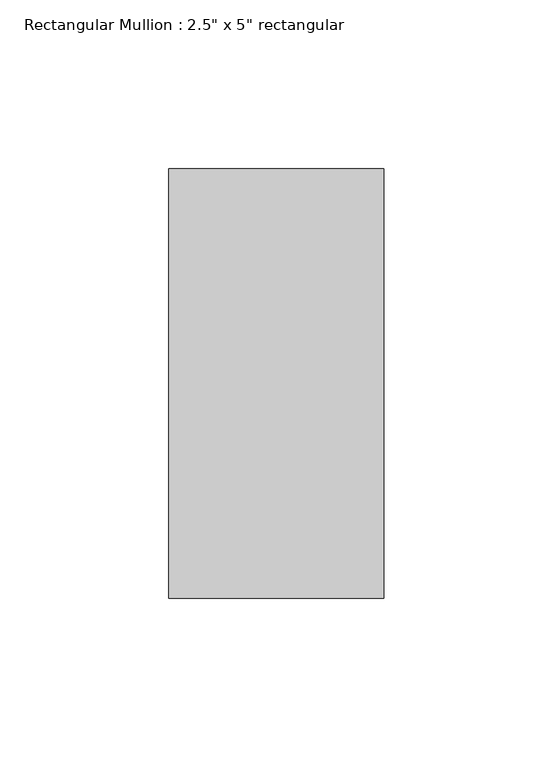
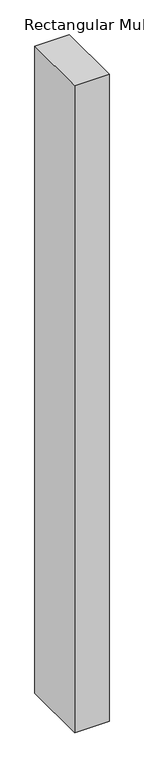
"""IFC4 building model written with IfcOpenShell, lengths in millimetres: member geometry."""

from ifc_helpers import new_model, si_unit, frame, origin, place, context, project, spatial, polyline, outline, extrude, source, transform, mapped, element, save


def member_76223ac8(model_context):
    return source(origin(), model_context, "Body", "SweptSolid", [
        extrude(outline(polyline([(31.75, 63.5), (31.75, -63.5), (-31.75, -63.5), (-31.75, 63.5), (31.75, 63.5)])), frame((0.0, 0.0, -1263.65), z_axis=(0.0, 0.0, 1.0), x_axis=(1.0, 0.0, 0.0)), (0.0, 0.0, 1.0), 1263.65),
    ])


if __name__ == "__main__":
    model = new_model("IFC4")
    model_context = context("Model", 3, world=origin())
    ifc_project = project(units=[si_unit("LENGTHUNIT", "METRE", prefix="MILLI")], contexts=[model_context])
    site = spatial("IfcSite", under=ifc_project)
    building = spatial("IfcBuilding", under=site)
    placement = place(None, origin())
    member_shape = member_76223ac8(model_context)
    element("IfcMember", 1, ObjectType="Rectangular Mullion : 2.5\" x 5\" rectangular", at=placement, inside=building, context=model_context, shape_type="MappedRepresentation", body=[
        mapped(member_shape, transform((0.0, 0.0, 0.0), x_axis=(1.0, 0.0, 0.0), y_axis=(0.0, 1.0, 0.0), z_axis=(0.0, 0.0, 1.0))),
    ])
    save(model, "model.ifc")

# Revit data of these elements
# Type "Rectangular Mullion : 2.5\" x 5\" rectangular"
#   built-in parameter 1007304 = 0.416667 (stored number, unit not read)
#   built-in parameter 1007301 = 0.104167 (stored number, unit not read)
#   built-in parameter 1007300 = 0.104167 (stored number, unit not read)
# Element 1 (IfcMember, "Rectangular Mullion : 2.5\" x 5\" rectangular")
#   Materials on its faces: "Metal - Aluminum"
# Materials
#   "Metal - Aluminum": class "Metal", colour RGB 140 140 140, transparency 0
